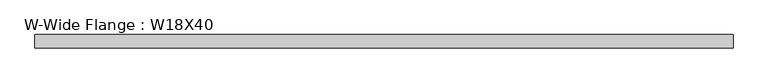
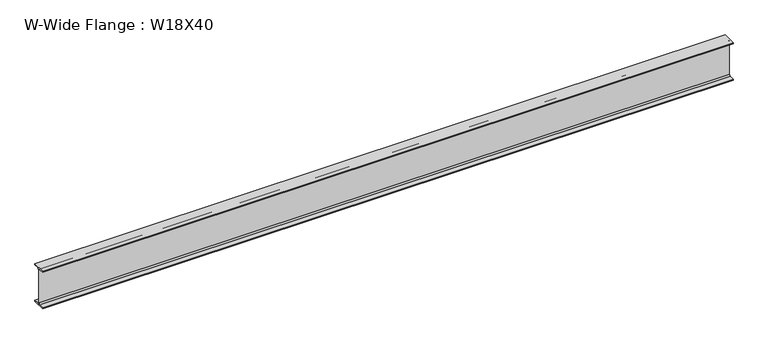
"""IFC4 building model written with IfcOpenShell, lengths in millimetres: beam geometry, W-Wide Flange : W18X40."""

import ifcopenshell
import ifcopenshell.guid

model = None  # the IFC model being written
_history = None  # IfcOwnerHistory: only IFC2X3 demands one
_inside = {}  # id of a spatial element -> (the spatial element, [elements in it])
_under = {}  # id of a project, library or spatial element -> (it, [spatial elements below it])
_declared = {}  # id of a project -> (the project, [libraries it declares])
_typed = {}  # id of a type object -> (the type object, [elements of that type])
_made_of = {}  # id of a material, layer set ... -> (it, [elements and type objects made of it])


def new_model(schema):
    """Start an empty IFC model of exactly this schema.

    Asked for "IFC4X3", IfcOpenShell would pick the latest addendum, in which some entities
    have other attributes; the version numbers below select the first issue.
    IFC2X3 requires an IfcOwnerHistory on every rooted entity: one is made here for all.
    """
    global model, _history
    if schema == "IFC4X3":
        model = ifcopenshell.file(schema_version=(4, 3, 0, 0))
    else:
        model = ifcopenshell.file(schema=schema)
    _inside.clear()
    _under.clear()
    _declared.clear()
    _typed.clear()
    _made_of.clear()
    _history = None
    if model.schema == "IFC2X3":
        org = make("IfcOrganization", Name="unknown")
        user = make(
            "IfcPersonAndOrganization",
            ThePerson=make("IfcPerson", FamilyName="unknown"),
            TheOrganization=org,
        )
        app = make(
            "IfcApplication",
            ApplicationDeveloper=org,
            Version="unknown",
            ApplicationFullName="unknown",
            ApplicationIdentifier="unknown",
        )
        _history = make(
            "IfcOwnerHistory",
            OwningUser=user,
            OwningApplication=app,
            ChangeAction="ADDED",
            CreationDate=0,
        )
    return model


def make(cls, **values):
    """One entity of the class cls with the attributes given. An attribute that is None is left unset."""
    return model.create_entity(
        cls, **{name: value for name, value in values.items() if value is not None}
    )


def rooted(cls, **values):
    """An entity with a GlobalId (a new one), such as an element, a storey or a relation."""
    return make(cls, GlobalId=ifcopenshell.guid.new(), OwnerHistory=_history, **values)


def si_unit(unit_type, name, prefix=None):
    """IfcSIUnit, for example si_unit("LENGTHUNIT", "METRE", prefix="MILLI")."""
    return make("IfcSIUnit", UnitType=unit_type, Prefix=prefix, Name=name)


def assignment(units):
    """IfcUnitAssignment: the units of a project."""
    return None if units is None else make("IfcUnitAssignment", Units=units)


def point(xyz):
    """IfcCartesianPoint."""
    return None if xyz is None else make("IfcCartesianPoint", Coordinates=xyz)


def direction(xyz):
    """IfcDirection."""
    return None if xyz is None else make("IfcDirection", DirectionRatios=xyz)


def frame(location, z_axis=None, x_axis=None):
    """IfcAxis2Placement3D, a coordinate frame: its origin and axes. An axis left out is left unset."""
    return make(
        "IfcAxis2Placement3D",
        Location=point(location),
        Axis=direction(z_axis),
        RefDirection=direction(x_axis),
    )


def frame_2d(location, x_axis=None):
    """IfcAxis2Placement2D, a coordinate frame in the plane: its origin and x axis."""
    return make(
        "IfcAxis2Placement2D", Location=point(location), RefDirection=direction(x_axis)
    )


def origin():
    """The frame at (0, 0, 0) with its axes left unset."""
    return frame((0.0, 0.0, 0.0))


def place(relative_to, where):
    """IfcLocalPlacement: puts the frame where relative to a parent placement (None: the world)."""
    return make(
        "IfcLocalPlacement", PlacementRelTo=relative_to, RelativePlacement=where
    )


def context(
    kind, dimensions, precision=None, world=None, true_north=None, identifier=None
):
    """IfcGeometricRepresentationContext, for example the 3D "Model" context."""
    return make(
        "IfcGeometricRepresentationContext",
        ContextIdentifier=identifier,
        ContextType=kind,
        CoordinateSpaceDimension=dimensions,
        Precision=precision,
        WorldCoordinateSystem=world,
        TrueNorth=true_north,
    )


def project(units=None, contexts=None):
    """IfcProject with its units and contexts."""
    return rooted(
        "IfcProject",
        Name="project",
        RepresentationContexts=contexts,
        UnitsInContext=assignment(units),
    )


def spatial(cls, under=None, at=None, **own):
    """A site, building, storey or space (cls), placed at a placement, below another one or the project."""
    s = rooted(cls, ObjectPlacement=at, **own)
    if under is not None:
        _under.setdefault(under.id(), (under, []))[1].append(s)
    return s


def polyline(points):
    """IfcPolyline through the points."""
    return make("IfcPolyline", Points=[point(p) for p in points])


def circle_curve(where, radius):
    """IfcCircle in the frame where."""
    return make("IfcCircle", Position=where, Radius=radius)


def trimmed(basis, trim1, trim2, sense, master):
    """IfcTrimmedCurve: the piece of a basis curve between two trims."""
    return make(
        "IfcTrimmedCurve",
        BasisCurve=basis,
        Trim1=trim1,
        Trim2=trim2,
        SenseAgreement=sense,
        MasterRepresentation=master,
    )


def segment(curve, same_sense, transition):
    """IfcCompositeCurveSegment."""
    return make(
        "IfcCompositeCurveSegment",
        Transition=transition,
        SameSense=same_sense,
        ParentCurve=curve,
    )


def composite_curve(segments, self_intersect=None):
    """IfcCompositeCurve: segments joined end to end."""
    return make("IfcCompositeCurve", Segments=segments, SelfIntersect=self_intersect)


def outline(outer, holes=None, kind="AREA"):
    """IfcArbitraryClosedProfileDef: a profile drawn as a closed curve; with holes, ...WithVoids."""
    if holes is None:
        return make("IfcArbitraryClosedProfileDef", ProfileType=kind, OuterCurve=outer)
    return make(
        "IfcArbitraryProfileDefWithVoids",
        ProfileType=kind,
        OuterCurve=outer,
        InnerCurves=holes,
    )


def extrude(swept, where, along, depth):
    """IfcExtrudedAreaSolid: the profile swept, set in the frame where, extruded along a direction by depth."""
    return make(
        "IfcExtrudedAreaSolid",
        SweptArea=swept,
        Position=where,
        ExtrudedDirection=direction(along),
        Depth=depth,
    )


def shape(context_of_items, identifier, shape_type, items):
    """IfcShapeRepresentation: the items that make up one representation, for example the "Body"."""
    return make(
        "IfcShapeRepresentation",
        ContextOfItems=context_of_items,
        RepresentationIdentifier=identifier,
        RepresentationType=shape_type,
        Items=items,
    )


def source(mapping_origin, context_of_items, identifier, shape_type, items):
    """IfcRepresentationMap: a shape defined once, which mapped items show again and again."""
    return make(
        "IfcRepresentationMap",
        MappingOrigin=mapping_origin,
        MappedRepresentation=shape(context_of_items, identifier, shape_type, items),
    )


def transform(
    local_origin,
    x_axis=None,
    y_axis=None,
    z_axis=None,
    scale=None,
    scale2=None,
    scale3=None,
    uniform=True,
):
    """IfcCartesianTransformationOperator3D, or its non-uniform kind. x_axis, y_axis, z_axis: its Axis1, 2, 3."""
    if uniform:
        return make(
            "IfcCartesianTransformationOperator3D",
            Axis1=direction(x_axis),
            Axis2=direction(y_axis),
            LocalOrigin=point(local_origin),
            Scale=scale,
            Axis3=direction(z_axis),
        )
    return make(
        "IfcCartesianTransformationOperator3DnonUniform",
        Axis1=direction(x_axis),
        Axis2=direction(y_axis),
        LocalOrigin=point(local_origin),
        Scale=scale,
        Axis3=direction(z_axis),
        Scale2=scale2,
        Scale3=scale3,
    )


def mapped(mapping_source, mapping_target):
    """IfcMappedItem: shows the shape of a source again, moved by a transform."""
    return make(
        "IfcMappedItem", MappingSource=mapping_source, MappingTarget=mapping_target
    )


def made_of(thing, what):
    """Note that an element or type object is made of a material, layer set ...; save() writes the relation."""
    if what is not None:
        _made_of.setdefault(what.id(), (what, []))[1].append(thing)
    return thing


def element(
    cls,
    number,
    at=None,
    inside=None,
    cuts=None,
    type_object=None,
    material=None,
    context=None,
    identifier="Body",
    shape_type=None,
    held_by="IfcProductDefinitionShape",
    body=None,
    shapes=None,
    **own,
):
    """One element of the class cls, such as IfcWall. Its Tag is "e" and its number.

    at: its placement. inside: the storey or other place that contains it. cuts: it is an
    opening in that element (IfcRelVoidsElement). A single representation is given by context,
    identifier, shape_type and body (its items); several are given by shapes. held_by: the class
    of the entity that holds the representations. save() writes the other relations.
    """
    e = rooted(cls, Tag="e%d" % number, ObjectPlacement=at, **own)
    if body is not None:
        shapes = [shape(context, identifier, shape_type, body)]
    if shapes is not None:
        e.Representation = make(held_by, Representations=shapes)
    if inside is not None:
        _inside.setdefault(inside.id(), (inside, []))[1].append(e)
    if cuts is not None:
        rooted(
            "IfcRelVoidsElement", RelatingBuildingElement=cuts, RelatedOpeningElement=e
        )
    if type_object is not None:
        _typed.setdefault(type_object.id(), (type_object, []))[1].append(e)
    return made_of(e, material)


def aggregate(whole, parts):
    """IfcRelAggregates: a whole, such as a stair, and the parts it consists of."""
    return rooted("IfcRelAggregates", RelatingObject=whole, RelatedObjects=parts)


def save(model, path):
    """Write the relations noted so far, then the file.

    IfcRelAggregates (storeys below a building ...), IfcRelContainedInSpatialStructure (elements
    in a storey), IfcRelDefinesByType, IfcRelAssociatesMaterial and IfcRelDeclares: one each for
    every whole, place, type object, material and project.
    """
    for whole, parts in _under.values():
        aggregate(whole, parts)
    for where, things in _inside.values():
        rooted(
            "IfcRelContainedInSpatialStructure",
            RelatedElements=things,
            RelatingStructure=where,
        )
    for kind, things in _typed.values():
        rooted("IfcRelDefinesByType", RelatedObjects=things, RelatingType=kind)
    for what, things in _made_of.values():
        rooted("IfcRelAssociatesMaterial", RelatedObjects=things, RelatingMaterial=what)
    for by, libraries in _declared.values():
        rooted("IfcRelDeclares", RelatingContext=by, RelatedDefinitions=libraries)
    model.write(path)


def w_wide_flange_w18x40_d8d7ebc0(model_context):
    return source(origin(), model_context, "Body", "SweptSolid", [
        extrude(outline(composite_curve([segment(polyline([(76.454, -213.995), (76.454, -227.33), (-76.454, -227.33), (-76.454, -213.995), (-20.828, -213.995)]), True, "CONTINUOUS"), segment(trimmed(circle_curve(frame_2d((-20.828, -197.1675)), 16.8275), [point((-20.828, -213.995))], [point((-4.0005, -197.1675))], True, "CARTESIAN"), True, "CONTINUOUS"), segment(polyline([(-4.0005, -197.1675), (-4.0005, 197.1675)]), True, "CONTINUOUS"), segment(trimmed(circle_curve(frame_2d((-20.828, 197.1675)), 16.8275), [point((-4.0005, 197.1675))], [point((-20.828, 213.995))], True, "CARTESIAN"), True, "CONTINUOUS"), segment(polyline([(-20.828, 213.995), (-76.454, 213.995), (-76.454, 227.33), (76.454, 227.33), (76.454, 213.995), (20.828, 213.995)]), True, "CONTINUOUS"), segment(trimmed(circle_curve(frame_2d((20.828, 197.1675)), 16.8275), [point((20.828, 213.995))], [point((4.0005, 197.1675))], True, "CARTESIAN"), True, "CONTINUOUS"), segment(polyline([(4.0005, 197.1675), (4.0005, -197.1675)]), True, "CONTINUOUS"), segment(trimmed(circle_curve(frame_2d((20.828, -197.1675)), 16.8275), [point((4.0005, -197.1675))], [point((20.828, -213.995))], True, "CARTESIAN"), True, "CONTINUOUS"), segment(polyline([(20.828, -213.995), (76.454, -213.995)]), True, "CONTINUOUS")], self_intersect=False)), frame((-3923.03, 0.0, 0.0), z_axis=(1.0, 0.0, 0.0), x_axis=(0.0, 1.0, 0.0)), (0.0, 0.0, 1.0), 7902.8925),
    ])


if __name__ == "__main__":
    model = new_model("IFC4")
    model_context = context("Model", 3, world=origin())
    ifc_project = project(units=[si_unit("LENGTHUNIT", "METRE", prefix="MILLI")], contexts=[model_context])
    site = spatial("IfcSite", under=ifc_project)
    building = spatial("IfcBuilding", under=site)
    placement = place(None, origin())
    w_wide_flange_w18x40_shape = w_wide_flange_w18x40_d8d7ebc0(model_context)
    element("IfcBeam", 1, ObjectType="W-Wide Flange : W18X40", at=placement, inside=building, context=model_context, shape_type="MappedRepresentation", body=[
        mapped(w_wide_flange_w18x40_shape, transform((0.0, 0.0, 0.0), x_axis=(1.0, 0.0, 0.0), y_axis=(0.0, 1.0, 0.0), z_axis=(0.0, 0.0, 1.0))),
    ])
    save(model, "model.ifc")

# Revit data of these elements
# Type "W-Wide Flange : W18X40"
#   Assembly Code = "B10"
#   W = 40
#   Length [instance default] = 5' - 0"
#   bf = 0' - 6.02"
#   d = 1' - 5.9"
#   k = 0' - 1 3/16"
#   k2 = 0' - 0.6625"
#   tf = 0' - 0.525"
#   tw = 0' - 0.315"
#   A = 0.0819444 SF
#   Structural Material [instance default] = Steel ASTM A992
# Element 1 (IfcBeam, "W-Wide Flange : W18X40")
#   Materials on its faces: "Steel ASTM A992"
# Materials
#   "Steel ASTM A992": class "Metal", colour RGB 199 199 199, transparency 0, Description = "Structural steel 50ksi", Cost = 0
